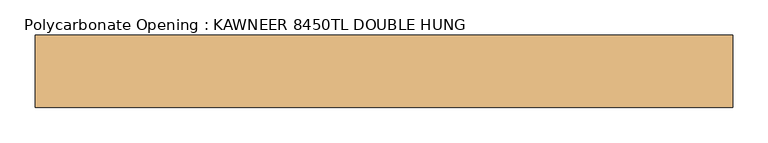
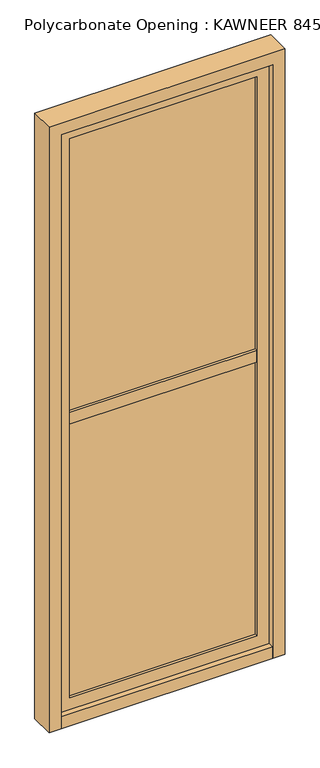
"""IFC4 building model written with IfcOpenShell, lengths in millimetres: door geometry, Polycarbonate Opening : KAWNEER 8450TL DOUBLE HUNG."""

from ifc_helpers import new_model, si_unit, frame, origin, origin_with_axes, place, context, project, spatial, polyline, outline, extrude, source, transform, mapped, element, save


def polycarbonate_opening_kawneer_8450tl_double_hung_ed50e2d1(model_context):
    return source(origin(), model_context, "Body", "SweptSolid", [
        extrude(outline(polyline([(440.1908884, 12.7), (440.1908884, -12.7), (-440.1908884, -12.7), (-440.1908884, 12.7), (440.1908884, 12.7)])), frame((0.0, 0.0, 50.8), z_axis=(0.0, 0.0, 1.0), x_axis=(1.0, 0.0, 0.0)), (0.0, 0.0, 1.0), 2561.1710618),
        extrude(outline(polyline([(2611.9710618, -440.1908884), (0.0, -440.1908884), (0.0, 440.1908884), (2611.9710618, 440.1908884), (2611.9710618, -440.1908884)]), holes=[polyline([(101.6, 389.3908884), (101.6, -389.3908884), (2561.1710618, -389.3908884), (2561.1710618, 389.3908884), (101.6, 389.3908884)])]), frame((0.0, -25.4, 0.0), z_axis=(0.0, 1.0, 0.0), x_axis=(0.0, 0.0, 1.0)), (0.0, 0.0, 1.0), 50.8),
        extrude(outline(polyline([(2662.7710618, 490.9908884), (2662.7710618, -490.9908884), (0.0, -490.9908884), (0.0, -440.1908884), (2611.9710618, -440.1908884), (2611.9710618, 440.1908884), (0.0, 440.1908884), (0.0, 490.9908884), (2662.7710618, 490.9908884)])), frame((0.0, -50.8, 0.0), z_axis=(0.0, 1.0, 0.0), x_axis=(0.0, 0.0, 1.0)), (0.0, 0.0, 1.0), 101.6),
        extrude(outline(polyline([(389.3908884, 25.4), (389.3908884, -25.4), (-389.3908884, -25.4), (-389.3908884, 25.4), (389.3908884, 25.4)])), frame((0.0, 0.0, 1305.9855309), z_axis=(0.0, 0.0, 1.0), x_axis=(1.0, 0.0, 0.0)), (0.0, 0.0, 1.0), 50.8),
        extrude(outline(polyline([(440.1908884, 50.8), (440.1908884, -50.8), (-440.1908884, -50.8), (-440.1908884, 50.8), (440.1908884, 50.8)])), origin_with_axes(), (0.0, 0.0, 1.0), 50.8),
    ])


if __name__ == "__main__":
    model = new_model("IFC4")
    model_context = context("Model", 3, world=origin())
    ifc_project = project(units=[si_unit("LENGTHUNIT", "METRE", prefix="MILLI")], contexts=[model_context])
    site = spatial("IfcSite", under=ifc_project)
    building = spatial("IfcBuilding", under=site)
    placement = place(None, origin())
    polycarbonate_opening_kawneer_8450tl_double_hung_shape = polycarbonate_opening_kawneer_8450tl_double_hung_ed50e2d1(model_context)
    element("IfcDoor", 1, ObjectType="Polycarbonate Opening : KAWNEER 8450TL DOUBLE HUNG", at=placement, inside=building, context=model_context, shape_type="MappedRepresentation", body=[
        mapped(polycarbonate_opening_kawneer_8450tl_double_hung_shape, transform((0.0, 0.0, 0.0), x_axis=(1.0, 0.0, 0.0), y_axis=(0.0, 1.0, 0.0), z_axis=(0.0, 0.0, 1.0))),
    ])
    save(model, "model.ifc")

# Revit data of these elements
# Type "Polycarbonate Opening : KAWNEER 8450TL DOUBLE HUNG"
#   Type Mark = "59"
#   OD_DS_Door_Material = "ALUM./GLAZING"
#   OD_DS_Door_Type = "STOREFRONT - DOUBLE HUNG WINDOW"
#   OD_DS_Lockset = "POLE OPERATOR HARDWARE FOR TOP SASH; BOTTOM SASH MECHANICALLY FIXED"
#   Analytic Construction = "<None>"
#   offset [instance default] = 0' - 2"
#   Stile = 0' - 2"
#   Mullion Width = 0' - 2"
#   Mullion Depth = 0' - 4"
#   Opening Size [instance default] = 5' - 1.50212"
#   Door Width [instance default] = 5' - 1.50212"
#   Window ON/OFF = no
#   Door On/Off = yes
#   Mullion Material = DOUBLE HUNG (CLEAR ANODIZED ALUM) - TEMPERED INSULATED GLAZING (CARDINAL GLASS LoĒ²-240\nOR EQUIVALENT)
#   Glass Material = TEMPERED INSULATED GLAZING (CARDINAL GLASS LoĒ²-240\nOR EQUIVALENT)
#   Door Material = DOUBLE HUNG (CLEAR ANODIZED ALUM) - TEMPERED INSULATED GLAZING (CARDINAL GLASS LoĒ²-240\nOR EQUIVALENT)
# Element 1 (IfcDoor, "Polycarbonate Opening : KAWNEER 8450TL DOUBLE HUNG")
#   offset = 0' - 0"
#   Materials on its faces: "DOUBLE HUNG (CLEAR ANODIZED ALUM) - TEMPERED INSULATED GLAZING (CARDINAL GLASS LoĒ²-240\nOR EQUIVALENT)", "TEMPERED INSULATED GLAZING (CARDINAL GLASS LoĒ²-240\nOR EQUIVALENT)"
# Materials
#   "DOUBLE HUNG (CLEAR ANODIZED ALUM) - TEMPERED INSULATED GLAZING (CARDINAL GLASS LoĒ²-240\nOR EQUIVALENT)": class "Metal", colour RGB 244 244 244, transparency 0, Description = "Aluminum 6061", Cost = 0
#   "TEMPERED INSULATED GLAZING (CARDINAL GLASS LoĒ²-240\nOR EQUIVALENT)": class "Glass", colour RGB 196 205 210, transparency 0.85, Description = "Soda Lime Glass", Cost = 0
